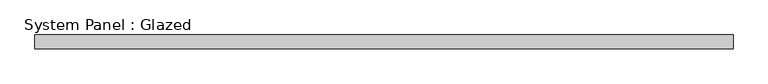
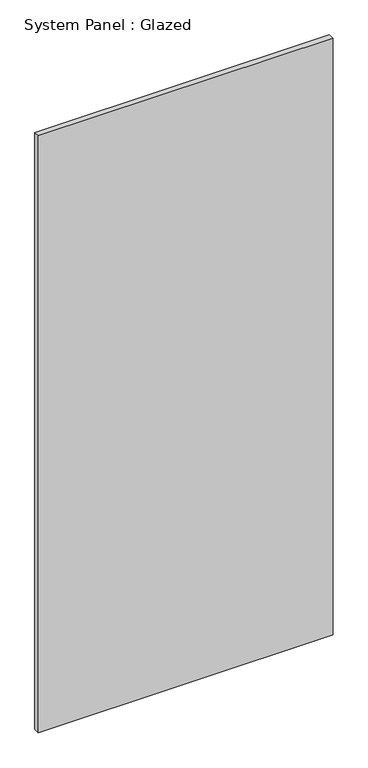
"""IFC4 building model written with IfcOpenShell, lengths in millimetres: plate geometry, System Panel : Glazed."""

from ifc_helpers import new_model, si_unit, origin, origin_with_axes, place, context, project, spatial, polyline, outline, extrude, source, transform, mapped, element, save


def system_panel_glazed_36e52168(model_context):
    return source(origin(), model_context, "Body", "SweptSolid", [
        extrude(outline(polyline([(651.3841819, 19.05), (-651.3841819, 19.05), (-651.3841819, 44.45), (651.3841819, 44.45), (651.3841819, 19.05)])), origin_with_axes(), (0.0, 0.0, 1.0), 2788.92),
    ])


if __name__ == "__main__":
    model = new_model("IFC4")
    model_context = context("Model", 3, world=origin())
    ifc_project = project(units=[si_unit("LENGTHUNIT", "METRE", prefix="MILLI")], contexts=[model_context])
    site = spatial("IfcSite", under=ifc_project)
    building = spatial("IfcBuilding", under=site)
    placement = place(None, origin())
    system_panel_glazed_shape = system_panel_glazed_36e52168(model_context)
    element("IfcPlate", 1, ObjectType="System Panel : Glazed", at=placement, inside=building, context=model_context, shape_type="MappedRepresentation", body=[
        mapped(system_panel_glazed_shape, transform((0.0, 0.0, 0.0), x_axis=(1.0, 0.0, 0.0), y_axis=(0.0, 1.0, 0.0), z_axis=(0.0, 0.0, 1.0))),
    ])
    save(model, "model.ifc")

# Revit data of these elements
# Type "System Panel : Glazed"
#   Construction Type Id = "GSP4R"
#   Analytic Construction = "1/8 in Pilkington single glazing"
#   Visual Light Transmittance = 0.9
#   Solar Heat Gain Coefficient = 0.86
#   Heat Transfer Coefficient (U) = 1.18115 BTU/(h·ft²·°F)
#   Define Thermal Properties by = 1
# Element 1 (IfcPlate, "System Panel : Glazed")
#   Materials on its faces: "Glass"
# Materials
#   "Glass": class "Glass", colour RGB 0 128 192, transparency 0.75, Description = "Soda Lime Glass", Cost = 0
